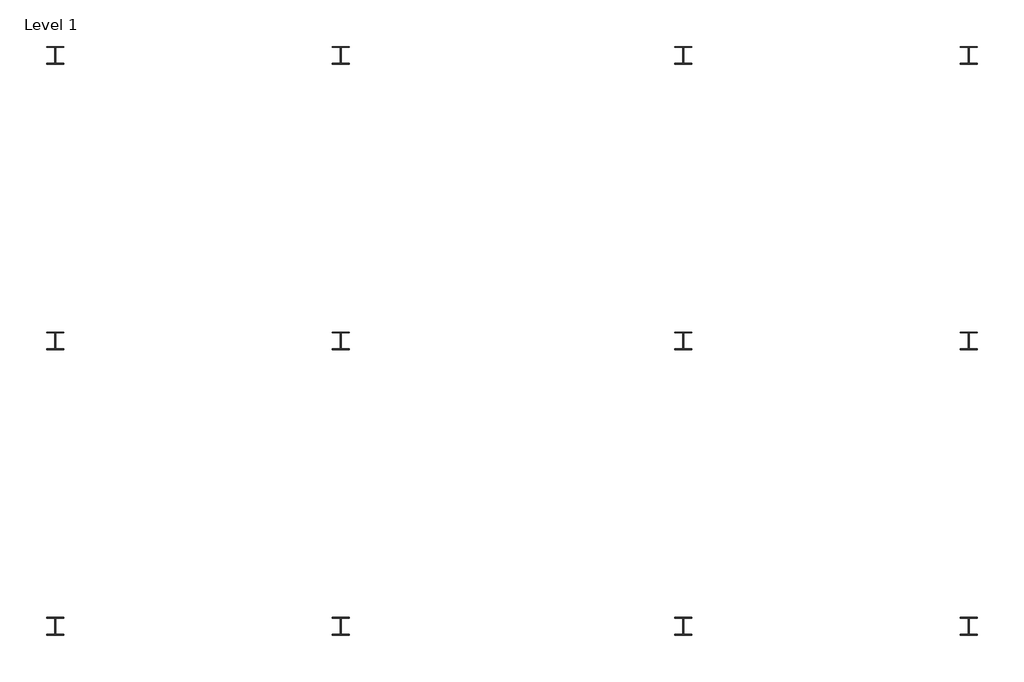
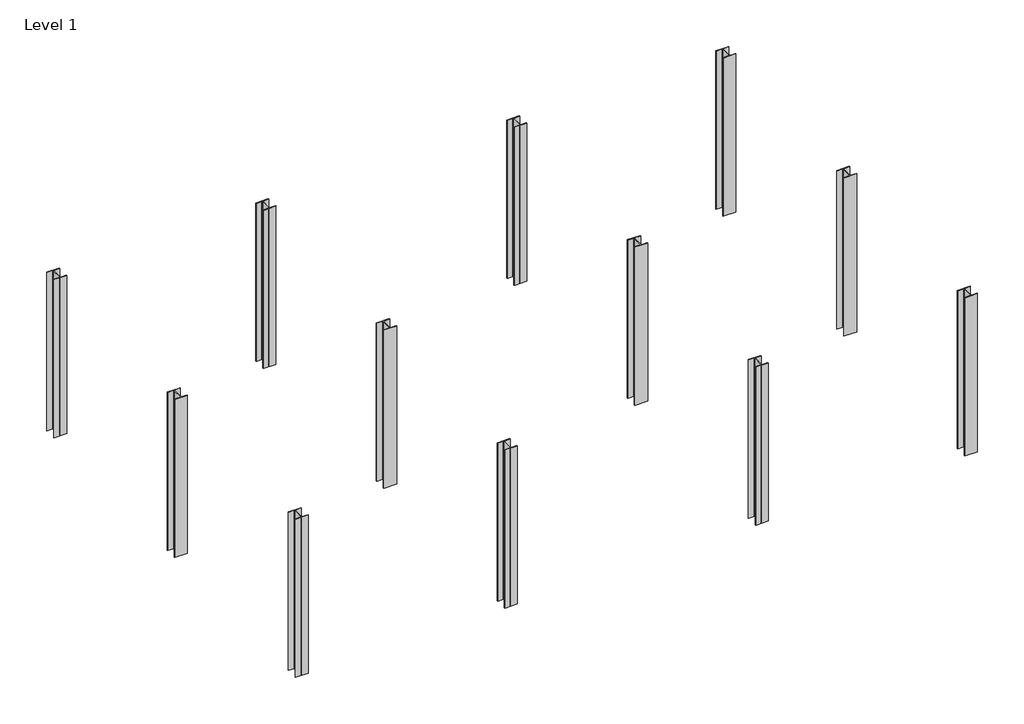
# One storey: 12 columns.
"""IFC4 building model written with IfcOpenShell, lengths in millimetres."""

from ifc_helpers import new_model, si_unit, point, frame_2d, origin, origin_with_axes, place, context, project, spatial, polyline, circle_curve, trimmed, segment, composite_curve, outline, extrude, element, save

model = new_model("IFC4")

# Units and contexts
model_context = context("Model", 3, world=origin())
ifc_project = project(units=[si_unit("LENGTHUNIT", "METRE", prefix="MILLI")], contexts=[model_context])

# Site, building, storey
site = spatial("IfcSite", under=ifc_project)
building = spatial("IfcBuilding", under=site)
storey = spatial("IfcBuildingStorey", under=building, Name="Level 1", Elevation=0.0)

# Columns
placement = place(None, origin())
element("IfcColumn", 1, ObjectType="UC-Universal Columns-Column : UC305x305x97", at=placement, inside=storey, context=model_context, shape_type="SweptSolid", body=[
    extrude(outline(composite_curve([segment(polyline([(152.65, 153.95), (152.65, 138.55), (20.15, 138.55)]), True, "CONTINUOUS"), segment(trimmed(circle_curve(frame_2d((20.15, 123.35)), 15.2), [point((20.15, 138.55))], [point((4.95, 123.35))], True, "CARTESIAN"), True, "CONTINUOUS"), segment(polyline([(4.95, 123.35), (4.95, -123.35)]), True, "CONTINUOUS"), segment(trimmed(circle_curve(frame_2d((20.15, -123.35)), 15.2), [point((4.95, -123.35))], [point((20.15, -138.55))], True, "CARTESIAN"), True, "CONTINUOUS"), segment(polyline([(20.15, -138.55), (152.65, -138.55), (152.65, -153.95), (-152.65, -153.95), (-152.65, -138.55), (-20.15, -138.55)]), True, "CONTINUOUS"), segment(trimmed(circle_curve(frame_2d((-20.15, -123.35)), 15.2), [point((-20.15, -138.55))], [point((-4.95, -123.35))], True, "CARTESIAN"), True, "CONTINUOUS"), segment(polyline([(-4.95, -123.35), (-4.95, 123.35)]), True, "CONTINUOUS"), segment(trimmed(circle_curve(frame_2d((-20.15, 123.35)), 15.2), [point((-4.95, 123.35))], [point((-20.15, 138.55))], True, "CARTESIAN"), True, "CONTINUOUS"), segment(polyline([(-20.15, 138.55), (-152.65, 138.55), (-152.65, 153.95), (152.65, 153.95)]), True, "CONTINUOUS")], self_intersect=False)), origin_with_axes(), (0.0, 0.0, 1.0), 4000.0),
])
element("IfcColumn", 2, ObjectType="UC-Universal Columns-Column : UC305x305x97", at=placement, inside=storey, context=model_context, shape_type="SweptSolid", body=[
    extrude(outline(composite_curve([segment(polyline([(5152.65, 153.95), (5152.65, 138.55), (5020.15, 138.55)]), True, "CONTINUOUS"), segment(trimmed(circle_curve(frame_2d((5020.15, 123.35)), 15.2), [point((5020.15, 138.55))], [point((5004.95, 123.35))], True, "CARTESIAN"), True, "CONTINUOUS"), segment(polyline([(5004.95, 123.35), (5004.95, -123.35)]), True, "CONTINUOUS"), segment(trimmed(circle_curve(frame_2d((5020.15, -123.35)), 15.2), [point((5004.95, -123.35))], [point((5020.15, -138.55))], True, "CARTESIAN"), True, "CONTINUOUS"), segment(polyline([(5020.15, -138.55), (5152.65, -138.55), (5152.65, -153.95), (4847.35, -153.95), (4847.35, -138.55), (4979.85, -138.55)]), True, "CONTINUOUS"), segment(trimmed(circle_curve(frame_2d((4979.85, -123.35)), 15.2), [point((4979.85, -138.55))], [point((4995.05, -123.35))], True, "CARTESIAN"), True, "CONTINUOUS"), segment(polyline([(4995.05, -123.35), (4995.05, 123.35)]), True, "CONTINUOUS"), segment(trimmed(circle_curve(frame_2d((4979.85, 123.35)), 15.2), [point((4995.05, 123.35))], [point((4979.85, 138.55))], True, "CARTESIAN"), True, "CONTINUOUS"), segment(polyline([(4979.85, 138.55), (4847.35, 138.55), (4847.35, 153.95), (5152.65, 153.95)]), True, "CONTINUOUS")], self_intersect=False)), origin_with_axes(), (0.0, 0.0, 1.0), 4000.0),
])
element("IfcColumn", 3, ObjectType="UC-Universal Columns-Column : UC305x305x97", at=placement, inside=storey, context=model_context, shape_type="SweptSolid", body=[
    extrude(outline(composite_curve([segment(polyline([(11152.65, 153.95), (11152.65, 138.55), (11020.15, 138.55)]), True, "CONTINUOUS"), segment(trimmed(circle_curve(frame_2d((11020.15, 123.35)), 15.2), [point((11020.15, 138.55))], [point((11004.95, 123.35))], True, "CARTESIAN"), True, "CONTINUOUS"), segment(polyline([(11004.95, 123.35), (11004.95, -123.35)]), True, "CONTINUOUS"), segment(trimmed(circle_curve(frame_2d((11020.15, -123.35)), 15.2), [point((11004.95, -123.35))], [point((11020.15, -138.55))], True, "CARTESIAN"), True, "CONTINUOUS"), segment(polyline([(11020.15, -138.55), (11152.65, -138.55), (11152.65, -153.95), (10847.35, -153.95), (10847.35, -138.55), (10979.85, -138.55)]), True, "CONTINUOUS"), segment(trimmed(circle_curve(frame_2d((10979.85, -123.35)), 15.2), [point((10979.85, -138.55))], [point((10995.05, -123.35))], True, "CARTESIAN"), True, "CONTINUOUS"), segment(polyline([(10995.05, -123.35), (10995.05, 123.35)]), True, "CONTINUOUS"), segment(trimmed(circle_curve(frame_2d((10979.85, 123.35)), 15.2), [point((10995.05, 123.35))], [point((10979.85, 138.55))], True, "CARTESIAN"), True, "CONTINUOUS"), segment(polyline([(10979.85, 138.55), (10847.35, 138.55), (10847.35, 153.95), (11152.65, 153.95)]), True, "CONTINUOUS")], self_intersect=False)), origin_with_axes(), (0.0, 0.0, 1.0), 4000.0),
])
element("IfcColumn", 4, ObjectType="UC-Universal Columns-Column : UC305x305x97", at=placement, inside=storey, context=model_context, shape_type="SweptSolid", body=[
    extrude(outline(composite_curve([segment(polyline([(16152.65, 153.95), (16152.65, 138.55), (16020.15, 138.55)]), True, "CONTINUOUS"), segment(trimmed(circle_curve(frame_2d((16020.15, 123.35)), 15.2), [point((16020.15, 138.55))], [point((16004.95, 123.35))], True, "CARTESIAN"), True, "CONTINUOUS"), segment(polyline([(16004.95, 123.35), (16004.95, -123.35)]), True, "CONTINUOUS"), segment(trimmed(circle_curve(frame_2d((16020.15, -123.35)), 15.2), [point((16004.95, -123.35))], [point((16020.15, -138.55))], True, "CARTESIAN"), True, "CONTINUOUS"), segment(polyline([(16020.15, -138.55), (16152.65, -138.55), (16152.65, -153.95), (15847.35, -153.95), (15847.35, -138.55), (15979.85, -138.55)]), True, "CONTINUOUS"), segment(trimmed(circle_curve(frame_2d((15979.85, -123.35)), 15.2), [point((15979.85, -138.55))], [point((15995.05, -123.35))], True, "CARTESIAN"), True, "CONTINUOUS"), segment(polyline([(15995.05, -123.35), (15995.05, 123.35)]), True, "CONTINUOUS"), segment(trimmed(circle_curve(frame_2d((15979.85, 123.35)), 15.2), [point((15995.05, 123.35))], [point((15979.85, 138.55))], True, "CARTESIAN"), True, "CONTINUOUS"), segment(polyline([(15979.85, 138.55), (15847.35, 138.55), (15847.35, 153.95), (16152.65, 153.95)]), True, "CONTINUOUS")], self_intersect=False)), origin_with_axes(), (0.0, 0.0, 1.0), 4000.0),
])
element("IfcColumn", 5, ObjectType="UC-Universal Columns-Column : UC305x305x97", at=placement, inside=storey, context=model_context, shape_type="SweptSolid", body=[
    extrude(outline(composite_curve([segment(polyline([(152.65, 5153.95), (152.65, 5138.55), (20.15, 5138.55)]), True, "CONTINUOUS"), segment(trimmed(circle_curve(frame_2d((20.15, 5123.35)), 15.2), [point((20.15, 5138.55))], [point((4.95, 5123.35))], True, "CARTESIAN"), True, "CONTINUOUS"), segment(polyline([(4.95, 5123.35), (4.95, 4876.65)]), True, "CONTINUOUS"), segment(trimmed(circle_curve(frame_2d((20.15, 4876.65)), 15.2), [point((4.95, 4876.65))], [point((20.15, 4861.45))], True, "CARTESIAN"), True, "CONTINUOUS"), segment(polyline([(20.15, 4861.45), (152.65, 4861.45), (152.65, 4846.05), (-152.65, 4846.05), (-152.65, 4861.45), (-20.15, 4861.45)]), True, "CONTINUOUS"), segment(trimmed(circle_curve(frame_2d((-20.15, 4876.65)), 15.2), [point((-20.15, 4861.45))], [point((-4.95, 4876.65))], True, "CARTESIAN"), True, "CONTINUOUS"), segment(polyline([(-4.95, 4876.65), (-4.95, 5123.35)]), True, "CONTINUOUS"), segment(trimmed(circle_curve(frame_2d((-20.15, 5123.35)), 15.2), [point((-4.95, 5123.35))], [point((-20.15, 5138.55))], True, "CARTESIAN"), True, "CONTINUOUS"), segment(polyline([(-20.15, 5138.55), (-152.65, 5138.55), (-152.65, 5153.95), (152.65, 5153.95)]), True, "CONTINUOUS")], self_intersect=False)), origin_with_axes(), (0.0, 0.0, 1.0), 4000.0),
])
element("IfcColumn", 6, ObjectType="UC-Universal Columns-Column : UC305x305x97", at=placement, inside=storey, context=model_context, shape_type="SweptSolid", body=[
    extrude(outline(composite_curve([segment(polyline([(5152.65, 5153.95), (5152.65, 5138.55), (5020.15, 5138.55)]), True, "CONTINUOUS"), segment(trimmed(circle_curve(frame_2d((5020.15, 5123.35)), 15.2), [point((5020.15, 5138.55))], [point((5004.95, 5123.35))], True, "CARTESIAN"), True, "CONTINUOUS"), segment(polyline([(5004.95, 5123.35), (5004.95, 4876.65)]), True, "CONTINUOUS"), segment(trimmed(circle_curve(frame_2d((5020.15, 4876.65)), 15.2), [point((5004.95, 4876.65))], [point((5020.15, 4861.45))], True, "CARTESIAN"), True, "CONTINUOUS"), segment(polyline([(5020.15, 4861.45), (5152.65, 4861.45), (5152.65, 4846.05), (4847.35, 4846.05), (4847.35, 4861.45), (4979.85, 4861.45)]), True, "CONTINUOUS"), segment(trimmed(circle_curve(frame_2d((4979.85, 4876.65)), 15.2), [point((4979.85, 4861.45))], [point((4995.05, 4876.65))], True, "CARTESIAN"), True, "CONTINUOUS"), segment(polyline([(4995.05, 4876.65), (4995.05, 5123.35)]), True, "CONTINUOUS"), segment(trimmed(circle_curve(frame_2d((4979.85, 5123.35)), 15.2), [point((4995.05, 5123.35))], [point((4979.85, 5138.55))], True, "CARTESIAN"), True, "CONTINUOUS"), segment(polyline([(4979.85, 5138.55), (4847.35, 5138.55), (4847.35, 5153.95), (5152.65, 5153.95)]), True, "CONTINUOUS")], self_intersect=False)), origin_with_axes(), (0.0, 0.0, 1.0), 4000.0),
])
element("IfcColumn", 7, ObjectType="UC-Universal Columns-Column : UC305x305x97", at=placement, inside=storey, context=model_context, shape_type="SweptSolid", body=[
    extrude(outline(composite_curve([segment(polyline([(11152.65, 5153.95), (11152.65, 5138.55), (11020.15, 5138.55)]), True, "CONTINUOUS"), segment(trimmed(circle_curve(frame_2d((11020.15, 5123.35)), 15.2), [point((11020.15, 5138.55))], [point((11004.95, 5123.35))], True, "CARTESIAN"), True, "CONTINUOUS"), segment(polyline([(11004.95, 5123.35), (11004.95, 4876.65)]), True, "CONTINUOUS"), segment(trimmed(circle_curve(frame_2d((11020.15, 4876.65)), 15.2), [point((11004.95, 4876.65))], [point((11020.15, 4861.45))], True, "CARTESIAN"), True, "CONTINUOUS"), segment(polyline([(11020.15, 4861.45), (11152.65, 4861.45), (11152.65, 4846.05), (10847.35, 4846.05), (10847.35, 4861.45), (10979.85, 4861.45)]), True, "CONTINUOUS"), segment(trimmed(circle_curve(frame_2d((10979.85, 4876.65)), 15.2), [point((10979.85, 4861.45))], [point((10995.05, 4876.65))], True, "CARTESIAN"), True, "CONTINUOUS"), segment(polyline([(10995.05, 4876.65), (10995.05, 5123.35)]), True, "CONTINUOUS"), segment(trimmed(circle_curve(frame_2d((10979.85, 5123.35)), 15.2), [point((10995.05, 5123.35))], [point((10979.85, 5138.55))], True, "CARTESIAN"), True, "CONTINUOUS"), segment(polyline([(10979.85, 5138.55), (10847.35, 5138.55), (10847.35, 5153.95), (11152.65, 5153.95)]), True, "CONTINUOUS")], self_intersect=False)), origin_with_axes(), (0.0, 0.0, 1.0), 4000.0),
])
element("IfcColumn", 8, ObjectType="UC-Universal Columns-Column : UC305x305x97", at=placement, inside=storey, context=model_context, shape_type="SweptSolid", body=[
    extrude(outline(composite_curve([segment(polyline([(16152.65, 5153.95), (16152.65, 5138.55), (16020.15, 5138.55)]), True, "CONTINUOUS"), segment(trimmed(circle_curve(frame_2d((16020.15, 5123.35)), 15.2), [point((16020.15, 5138.55))], [point((16004.95, 5123.35))], True, "CARTESIAN"), True, "CONTINUOUS"), segment(polyline([(16004.95, 5123.35), (16004.95, 4876.65)]), True, "CONTINUOUS"), segment(trimmed(circle_curve(frame_2d((16020.15, 4876.65)), 15.2), [point((16004.95, 4876.65))], [point((16020.15, 4861.45))], True, "CARTESIAN"), True, "CONTINUOUS"), segment(polyline([(16020.15, 4861.45), (16152.65, 4861.45), (16152.65, 4846.05), (15847.35, 4846.05), (15847.35, 4861.45), (15979.85, 4861.45)]), True, "CONTINUOUS"), segment(trimmed(circle_curve(frame_2d((15979.85, 4876.65)), 15.2), [point((15979.85, 4861.45))], [point((15995.05, 4876.65))], True, "CARTESIAN"), True, "CONTINUOUS"), segment(polyline([(15995.05, 4876.65), (15995.05, 5123.35)]), True, "CONTINUOUS"), segment(trimmed(circle_curve(frame_2d((15979.85, 5123.35)), 15.2), [point((15995.05, 5123.35))], [point((15979.85, 5138.55))], True, "CARTESIAN"), True, "CONTINUOUS"), segment(polyline([(15979.85, 5138.55), (15847.35, 5138.55), (15847.35, 5153.95), (16152.65, 5153.95)]), True, "CONTINUOUS")], self_intersect=False)), origin_with_axes(), (0.0, 0.0, 1.0), 4000.0),
])
element("IfcColumn", 9, ObjectType="UC-Universal Columns-Column : UC305x305x97", at=placement, inside=storey, context=model_context, shape_type="SweptSolid", body=[
    extrude(outline(composite_curve([segment(polyline([(152.65, 10153.95), (152.65, 10138.55), (20.15, 10138.55)]), True, "CONTINUOUS"), segment(trimmed(circle_curve(frame_2d((20.15, 10123.35)), 15.2), [point((20.15, 10138.55))], [point((4.95, 10123.35))], True, "CARTESIAN"), True, "CONTINUOUS"), segment(polyline([(4.95, 10123.35), (4.95, 9876.65)]), True, "CONTINUOUS"), segment(trimmed(circle_curve(frame_2d((20.15, 9876.65)), 15.2), [point((4.95, 9876.65))], [point((20.15, 9861.45))], True, "CARTESIAN"), True, "CONTINUOUS"), segment(polyline([(20.15, 9861.45), (152.65, 9861.45), (152.65, 9846.05), (-152.65, 9846.05), (-152.65, 9861.45), (-20.15, 9861.45)]), True, "CONTINUOUS"), segment(trimmed(circle_curve(frame_2d((-20.15, 9876.65)), 15.2), [point((-20.15, 9861.45))], [point((-4.95, 9876.65))], True, "CARTESIAN"), True, "CONTINUOUS"), segment(polyline([(-4.95, 9876.65), (-4.95, 10123.35)]), True, "CONTINUOUS"), segment(trimmed(circle_curve(frame_2d((-20.15, 10123.35)), 15.2), [point((-4.95, 10123.35))], [point((-20.15, 10138.55))], True, "CARTESIAN"), True, "CONTINUOUS"), segment(polyline([(-20.15, 10138.55), (-152.65, 10138.55), (-152.65, 10153.95), (152.65, 10153.95)]), True, "CONTINUOUS")], self_intersect=False)), origin_with_axes(), (0.0, 0.0, 1.0), 4000.0),
])
element("IfcColumn", 10, ObjectType="UC-Universal Columns-Column : UC305x305x97", at=placement, inside=storey, context=model_context, shape_type="SweptSolid", body=[
    extrude(outline(composite_curve([segment(polyline([(5152.65, 10153.95), (5152.65, 10138.55), (5020.15, 10138.55)]), True, "CONTINUOUS"), segment(trimmed(circle_curve(frame_2d((5020.15, 10123.35)), 15.2), [point((5020.15, 10138.55))], [point((5004.95, 10123.35))], True, "CARTESIAN"), True, "CONTINUOUS"), segment(polyline([(5004.95, 10123.35), (5004.95, 9876.65)]), True, "CONTINUOUS"), segment(trimmed(circle_curve(frame_2d((5020.15, 9876.65)), 15.2), [point((5004.95, 9876.65))], [point((5020.15, 9861.45))], True, "CARTESIAN"), True, "CONTINUOUS"), segment(polyline([(5020.15, 9861.45), (5152.65, 9861.45), (5152.65, 9846.05), (4847.35, 9846.05), (4847.35, 9861.45), (4979.85, 9861.45)]), True, "CONTINUOUS"), segment(trimmed(circle_curve(frame_2d((4979.85, 9876.65)), 15.2), [point((4979.85, 9861.45))], [point((4995.05, 9876.65))], True, "CARTESIAN"), True, "CONTINUOUS"), segment(polyline([(4995.05, 9876.65), (4995.05, 10123.35)]), True, "CONTINUOUS"), segment(trimmed(circle_curve(frame_2d((4979.85, 10123.35)), 15.2), [point((4995.05, 10123.35))], [point((4979.85, 10138.55))], True, "CARTESIAN"), True, "CONTINUOUS"), segment(polyline([(4979.85, 10138.55), (4847.35, 10138.55), (4847.35, 10153.95), (5152.65, 10153.95)]), True, "CONTINUOUS")], self_intersect=False)), origin_with_axes(), (0.0, 0.0, 1.0), 4000.0),
])
element("IfcColumn", 11, ObjectType="UC-Universal Columns-Column : UC305x305x97", at=placement, inside=storey, context=model_context, shape_type="SweptSolid", body=[
    extrude(outline(composite_curve([segment(polyline([(11152.65, 10153.95), (11152.65, 10138.55), (11020.15, 10138.55)]), True, "CONTINUOUS"), segment(trimmed(circle_curve(frame_2d((11020.15, 10123.35)), 15.2), [point((11020.15, 10138.55))], [point((11004.95, 10123.35))], True, "CARTESIAN"), True, "CONTINUOUS"), segment(polyline([(11004.95, 10123.35), (11004.95, 9876.65)]), True, "CONTINUOUS"), segment(trimmed(circle_curve(frame_2d((11020.15, 9876.65)), 15.2), [point((11004.95, 9876.65))], [point((11020.15, 9861.45))], True, "CARTESIAN"), True, "CONTINUOUS"), segment(polyline([(11020.15, 9861.45), (11152.65, 9861.45), (11152.65, 9846.05), (10847.35, 9846.05), (10847.35, 9861.45), (10979.85, 9861.45)]), True, "CONTINUOUS"), segment(trimmed(circle_curve(frame_2d((10979.85, 9876.65)), 15.2), [point((10979.85, 9861.45))], [point((10995.05, 9876.65))], True, "CARTESIAN"), True, "CONTINUOUS"), segment(polyline([(10995.05, 9876.65), (10995.05, 10123.35)]), True, "CONTINUOUS"), segment(trimmed(circle_curve(frame_2d((10979.85, 10123.35)), 15.2), [point((10995.05, 10123.35))], [point((10979.85, 10138.55))], True, "CARTESIAN"), True, "CONTINUOUS"), segment(polyline([(10979.85, 10138.55), (10847.35, 10138.55), (10847.35, 10153.95), (11152.65, 10153.95)]), True, "CONTINUOUS")], self_intersect=False)), origin_with_axes(), (0.0, 0.0, 1.0), 4000.0),
])
element("IfcColumn", 12, ObjectType="UC-Universal Columns-Column : UC305x305x97", at=placement, inside=storey, context=model_context, shape_type="SweptSolid", body=[
    extrude(outline(composite_curve([segment(polyline([(16152.65, 10153.95), (16152.65, 10138.55), (16020.15, 10138.55)]), True, "CONTINUOUS"), segment(trimmed(circle_curve(frame_2d((16020.15, 10123.35)), 15.2), [point((16020.15, 10138.55))], [point((16004.95, 10123.35))], True, "CARTESIAN"), True, "CONTINUOUS"), segment(polyline([(16004.95, 10123.35), (16004.95, 9876.65)]), True, "CONTINUOUS"), segment(trimmed(circle_curve(frame_2d((16020.15, 9876.65)), 15.2), [point((16004.95, 9876.65))], [point((16020.15, 9861.45))], True, "CARTESIAN"), True, "CONTINUOUS"), segment(polyline([(16020.15, 9861.45), (16152.65, 9861.45), (16152.65, 9846.05), (15847.35, 9846.05), (15847.35, 9861.45), (15979.85, 9861.45)]), True, "CONTINUOUS"), segment(trimmed(circle_curve(frame_2d((15979.85, 9876.65)), 15.2), [point((15979.85, 9861.45))], [point((15995.05, 9876.65))], True, "CARTESIAN"), True, "CONTINUOUS"), segment(polyline([(15995.05, 9876.65), (15995.05, 10123.35)]), True, "CONTINUOUS"), segment(trimmed(circle_curve(frame_2d((15979.85, 10123.35)), 15.2), [point((15995.05, 10123.35))], [point((15979.85, 10138.55))], True, "CARTESIAN"), True, "CONTINUOUS"), segment(polyline([(15979.85, 10138.55), (15847.35, 10138.55), (15847.35, 10153.95), (16152.65, 10153.95)]), True, "CONTINUOUS")], self_intersect=False)), origin_with_axes(), (0.0, 0.0, 1.0), 4000.0),
])

save(model, "model.ifc")

# Revit data of these elements
# Project information
#   Project Issue Date = "Issue Date"
#   Project Status = "Project Status"
#   Client Name = "Owner"
#   Project Address = "Enter address here"
#   Project Name = "Project Name"
#   Project Number = "Project Number"
# Grids (mm)
#   "1": line (-3000, 0) -> (19000, 0)
#   "2": line (-3000, 5000) -> (19000, 5000)
#   "3": line (-3000, 10000) -> (19000, 10000)
#   "4": line (0, -3000) -> (0, 13000)
#   "5": line (5000, -3000) -> (5000, 13000)
#   "6": line (11000, -3000) -> (11000, 13000)
#   "7": line (16000, -3000) -> (16000, 13000)
# Type "UC-Universal Columns-Column : UC305x305x97"
#   Section Name Key = "UC305x305x97"
#   Width = 30.53 cm
#   Web Thickness = 0.99 cm
#   Web Fillet = 1.52 cm
#   Warping Constant = 1560000.0 cm⁶
#   Torsional Moment of Inertia = 91.20 cm⁴
#   Section Area = 123.0 cm²
#   Plastic Modulus weak axis = 726.0 cm³
#   Plastic Modulus strong axis = 1592.0 cm³
#   Nominal Weight = 96.8996 kgf/m
#   Moment of Inertia weak axis = 7308.00 cm⁴
#   Moment of Inertia strong axis = 22249.00 cm⁴
#   Height = 30.79 cm
#   Flange Thickness = 1.54 cm
#   Elastic Modulus weak axis = 479.0 cm³
#   Elastic Modulus strong axis = 1445.0 cm³
#   Centroid Vertical = 15.395 cm
#   Centroid Horizontal = 15.265 cm
#   Bolt Spacing = 14.0 cm
#   Structural Material [instance default] = Metal - Steel 43-275
#   Type Comments = ""
#   Assembly Code = ""
# Elements 1, 2, 3, 4, 5, 6, 7, 8, 9, 10, 11, 12 (IfcColumn, "UC-Universal Columns-Column : UC305x305x97")
#   Structural Material = Metal - Steel 43-275
#   Phase Created = New Construction
#   Materials on its faces: "Metal - Steel 43-275"
# Materials
#   "Metal - Steel 43-275": class "Metal", colour RGB 247 247 247, transparency 0, Cost = 0
